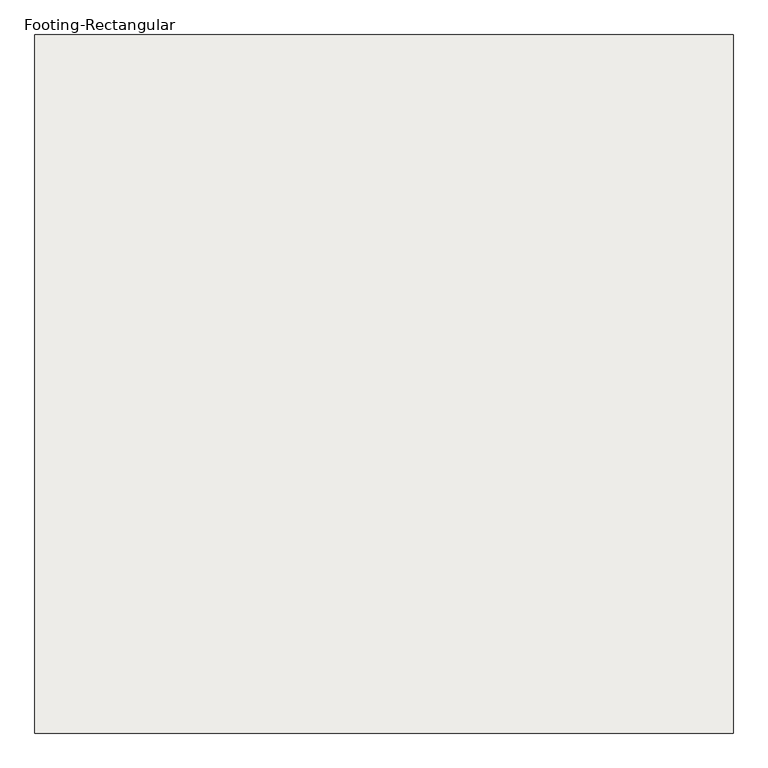
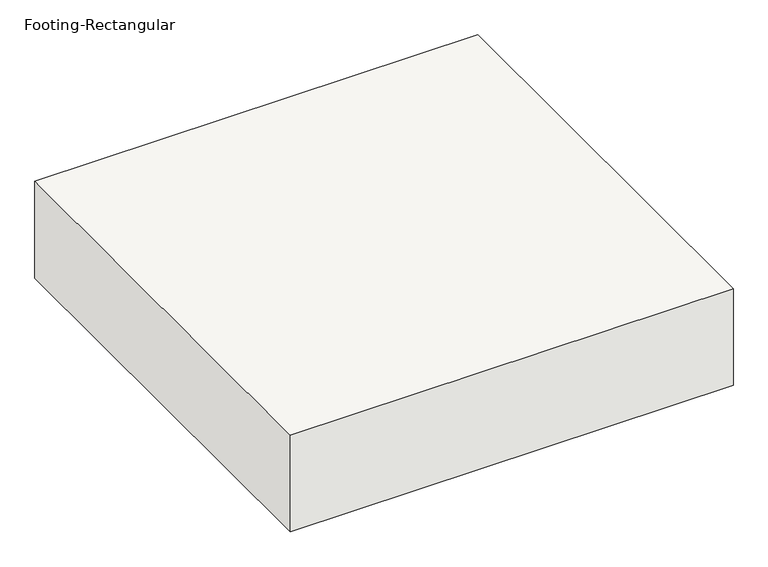
"""IFC4 building model written with IfcOpenShell, lengths in millimetres: slab geometry, Footing-Rectangular."""

from ifc_helpers import new_model, si_unit, frame, origin, place, context, project, spatial, polyline, outline, extrude, source, transform, mapped, element, save


def footing_rectangular_876cc71e(model_context):
    return source(origin(), model_context, "Body", "SweptSolid", [
        extrude(outline(polyline([(990.6, 990.6), (990.6, -990.6), (-990.6, -990.6), (-990.6, 990.6), (990.6, 990.6)])), frame((0.0, 0.0, -457.2), z_axis=(0.0, 0.0, 1.0), x_axis=(1.0, 0.0, 0.0)), (0.0, 0.0, 1.0), 457.2),
    ])


if __name__ == "__main__":
    model = new_model("IFC4")
    model_context = context("Model", 3, world=origin())
    ifc_project = project(units=[si_unit("LENGTHUNIT", "METRE", prefix="MILLI")], contexts=[model_context])
    site = spatial("IfcSite", under=ifc_project)
    building = spatial("IfcBuilding", under=site)
    placement = place(None, origin())
    footing_rectangular_shape = footing_rectangular_876cc71e(model_context)
    element("IfcSlab", 1, ObjectType="Footing-Rectangular : D 6.5' x 6.5' x 18\"", at=placement, inside=building, context=model_context, shape_type="MappedRepresentation", body=[
        mapped(footing_rectangular_shape, transform((0.0, 0.0, 0.0), x_axis=(1.0, 0.0, 0.0), y_axis=(0.0, 1.0, 0.0), z_axis=(0.0, 0.0, 1.0))),
    ])
    save(model, "model.ifc")

# Revit data of these elements
# Type "Footing-Rectangular : D 6.5' x 6.5' x 18\""
#   Assembly Code = "A1010100"
#   Width = 6' - 6"
#   Length = 6' - 6"
#   Foundation Thickness = 1' - 6"
#   Structural Material [instance default] = Concrete, Cast-in-Place gray
# Element 1 (IfcSlab, "Footing-Rectangular : D 6.5' x 6.5' x 18\"")
#   Materials on its faces: "Concrete, Cast-in-Place gray"
# Materials
#   "Concrete, Cast-in-Place gray": class "Concrete", colour RGB 192 192 192, transparency 0, Description = "Cast-in-place concrete", Cost = 0
